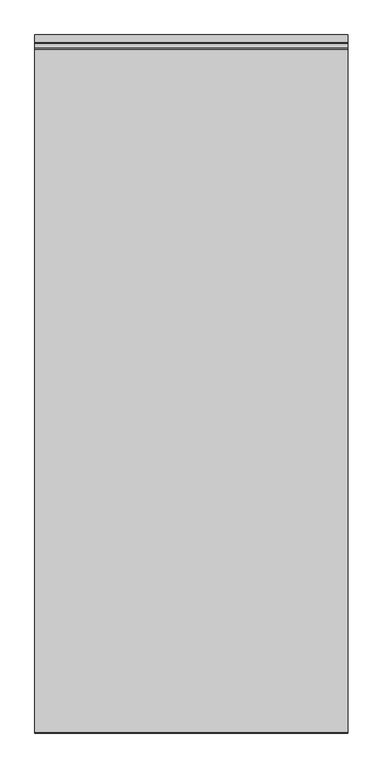
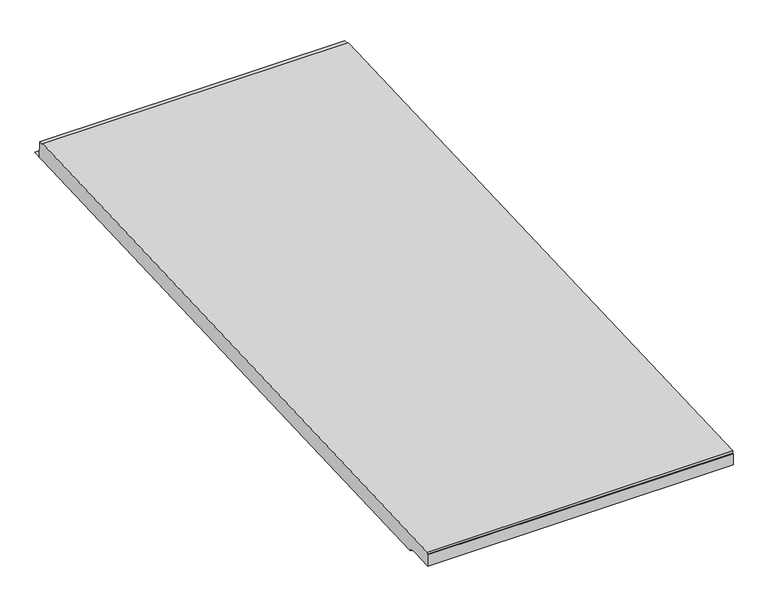
"""IFC4 building model written with IfcOpenShell, lengths in millimetres: proxy geometry, Generic Models 7:Generic Models 1:2:Generic Models 1:2 : Generic Models 7:Generic Models 1:337419:11 : Generic Models 7:Generic Models 1:2:Generic Models 1:2 : Generic Models 7:Generic Models 1:337419:306751."""

from ifc_helpers import new_model, si_unit, frame, origin, place, context, project, spatial, polyline, outline, extrude, source, transform, mapped, element, save


def generic_models_be7492b3(model_context):
    return source(origin(), model_context, "Body", "SweptSolid", [
        extrude(outline(polyline([(-568426.430308, 4390.492563), (-568407.8188757, 4365.8460002), (-568333.9629878, 4368.9233289), (-568323.3888294, 4115.1435284), (-568205.6913841, 4120.0475886), (-568205.6913841, 4116.8698337), (-578587.511845, 3684.2939812), (-578600.6413841, 3729.3727144), (-578603.2165864, 3731.9479167), (-578740.3413841, 3731.9479167), (-579068.9538841, 3718.2557292), (-579068.9538841, 3908.921022), (-579056.2717715, 3909.4494434), (-579057.8578953, 3947.5164135), (-568426.430308, 4390.492563)])), frame((591306.0367239, 0.0, 0.0), z_axis=(1.0, 0.0, 0.0), x_axis=(0.0, 1.0, 0.0)), (0.0, 0.0, 1.0), 4876.8),
    ])


if __name__ == "__main__":
    model = new_model("IFC4")
    model_context = context("Model", 3, world=origin())
    ifc_project = project(units=[si_unit("LENGTHUNIT", "METRE", prefix="MILLI")], contexts=[model_context])
    site = spatial("IfcSite", under=ifc_project)
    building = spatial("IfcBuilding", under=site)
    placement = place(None, origin())
    generic_models_shape = generic_models_be7492b3(model_context)
    element("IfcBuildingElementProxy", 1, Name="Generic Models 7:Generic Models 1:2:Generic Models 1:2 : Generic Models 7:Generic Models 1:337419:11 : Generic Models 7:Generic Models 1:2:Generic Models 1:2 : Generic Models 7:Generic Models 1:337419:306751", ObjectType="Generic Models 7:Generic Models 1:2:Generic Models 1:2 : Generic Models 7:Generic Models 1:337419:11 : Generic Models 7:Generic Models 1:2:Generic Models 1:2 : Generic Models 7:Generic Models 1:337419:306751", at=placement, inside=building, context=model_context, shape_type="MappedRepresentation", body=[
        mapped(generic_models_shape, transform((0.0, 0.0, 0.0), x_axis=(1.0, 0.0, 0.0), y_axis=(0.0, 1.0, 0.0), z_axis=(0.0, 0.0, 1.0))),
    ])
    save(model, "model.ifc")

# Revit data of these elements
# Type "Generic Models 7:Generic Models 1:2:Generic Models 1:2 : Generic Models 7:Generic Models 1:337419:11 : Generic Models 7:Generic Models 1:2:Generic Models 1:2 : Generic Models 7:Generic Models 1:337419:306751"
#   NameOverride = "Generic Models 7:Generic Models 1:2:Generic Models 1:2 : Generic Models 7:Generic Models 1:337419:306751"
#   ObjectTypeOverride = "Generic Models 1:2 : Generic Models 7:Generic Models 1:337419"
#   Reference = "Generic Models 1"
#   Tag = "306751"
# Element 1 (IfcBuildingElementProxy, "Generic Models 7:Generic Models 1:2:Generic Models 1:2 : Generic Models 7:Generic Models 1:337419:11 : Generic Models 7:Generic Models 1:2:Generic Models 1:2 : Generic Models 7:Generic Models 1:337419:306751")
#   Materials on its faces: "SIMPLE SAVER INSULATION WITH LINER - COLOR: BLACK"
# Materials
#   "SIMPLE SAVER INSULATION WITH LINER - COLOR: BLACK": class "Unassigned", colour RGB 158 92 175, transparency 0, Cost = 0
